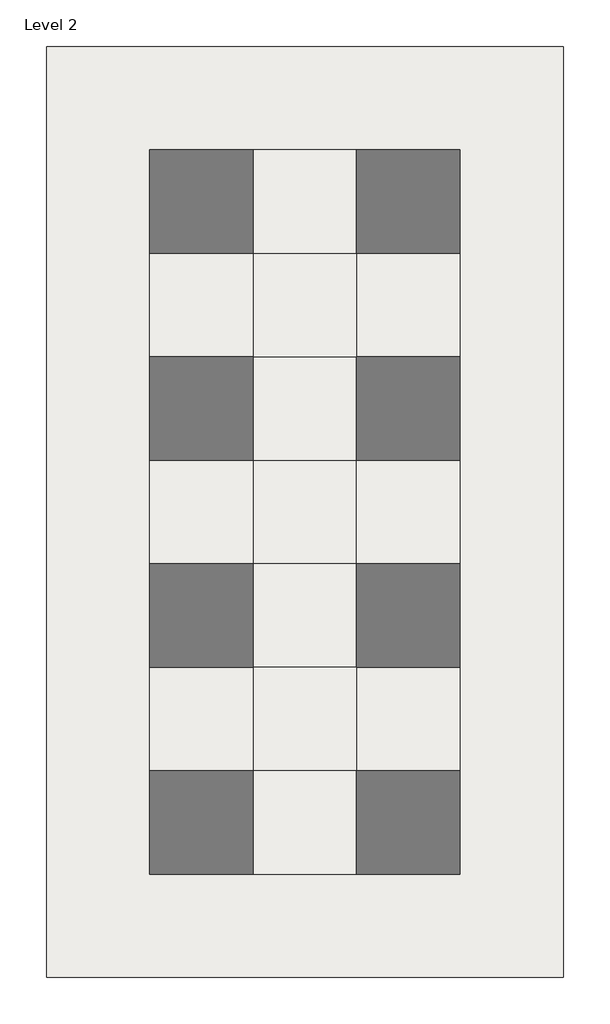
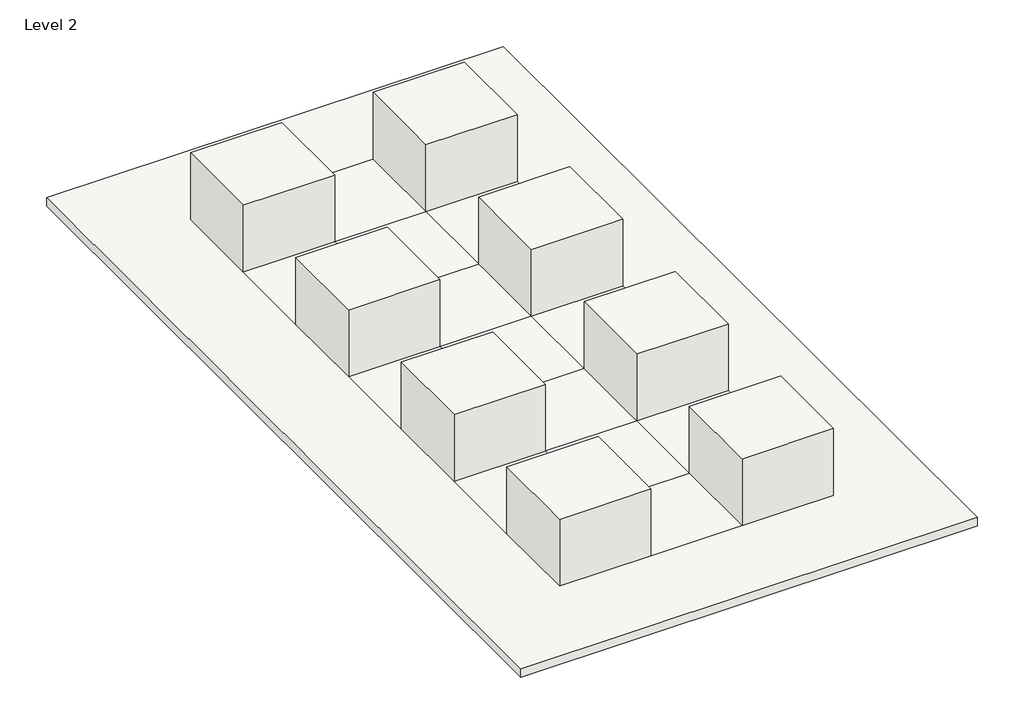
# One storey: 9 roofs.
# Revit data of these elements (continued)
# Materials (continued)
#   "Bauder_SeparationAndSlipLayer_BauderGREEN-PE-02": class "Unassigned", colour RGB 255 255 255, transparency 0, Mtrl_Author = "AM", Mtrl_AuthorizedBy = "bimstore", Mtrl_DistributedBy = "www.bimstore.co", Mtrl_AccessibilityPerformance = "n/a", Mtrl_AssetIdentifier = "Please record on commissioning", Mtrl_AssetType = "Fixed", Mtrl_BarCode = "Please record on commissioning", Mtrl_ClassificationName = "Uniclass2015", Mtrl_ClassificationValue = "n/a", Mtrl_CodePerformance = "n/a", Mtrl_Color = "n/a", Mtrl_Constituents = "n/a", Mtrl_CreatedBy = "technical@bauder.co.uk", Mtrl_CreatedOn = "2023-02-10 T00:00:00", Mtrl_DocumentationCertificates = "https://www.bimstore.co/products/intensive-green-roof-system/document/product-certificates", Mtrl_DocumentationInstallationGuide = "https://www.bimstore.co/products/intensive-green-roof-system/document/installation-guide", Mtrl_DocumentationLiterature = "https://www.bimstore.co/products/intensive-green-roof-system/document/product-literature", Mtrl_DocumentationMaintenance = "https://www.bimstore.co/products/intensive-green-roof-system/document/maintenance-information", Mtrl_DocumentationTechnical = "https://www.bimstore.co/products/intensive-green-roof-system/document/technical-data-sheet", Mtrl_DurationUnit = "Year", Mtrl_Features = "n/a", Mtrl_Finish = "n/a", Mtrl_Grade = "n/a", Mtrl_InstallationDate = "Please record on commissioning", Mtrl_ManufacturerName = "Bauder Ltd", Mtrl_Material = "n/a", Mtrl_ModelNumber = "BauderGREEN-PE-02", Mtrl_ModelReference = "Separation And Slip Layer", Mtrl_ProductionYear = "2023", Mtrl_ReferencedStandard = "n/a", Mtrl_Shape = "n/a", Mtrl_Size = "n/a", Mtrl_SpareParts = "n/a", Mtrl_TypeName = "BauderGREEN-PE-02", Mtrl_WarrantyDescription = "As part of Bauder system guarantee, per specification", Mtrl_WarrantyDurationUnit = "Year", Mtrl_WarrantyGuarantorLabor = "n/a", Mtrl_WarrantyGuarantorParts = "technical@bauder.co.uk", Mtrl_WarrantyStartDate = "Please record on commissioning", Mtrl_IfcExportAs = "IfcRoofType", Mtrl_IfcExportType = "FLAT_ROOF", Mtrl_BIMObjectName = "Bauder_SeparationAndSlipLayer_BauderGREEN-PE-02", Mtrl_NBSDescription = "n/a", Mtrl_NBSNote = "n/a", Mtrl_NBSObjectName = "n/a", Mtrl_NBSOfficeMasterTag = "n/a", Mtrl_NBSReference = "Q37", Mtrl_Ballast = "n/a", Mtrl_CarrierMembraneAttachment = "n/a", Mtrl_CarrierMembraneFixing = "n/a", Mtrl_CarrierMembraneType = "n/a", Mtrl_Certification = "Comply with GRO Green Roof Code of Practice and FLL Standards", Mtrl_DetailWorkAncillaryItems = "Detail as per project specific Bauder Specification", Mtrl_DetailWorkCoverStrips = "Detail as per project specific Bauder Specification", Mtrl_DetailWorkFlashings = "Detail as per project specific Bauder Specification", Mtrl_DetailWorkSkirtingsAndUpstands = "Detail as per project specific Bauder Specification", Mtrl_DetailWorkWeltedDrips = "Detail as per project specific Bauder Specification", Mtrl_EdgeRestraints = "Detail as per project specific Bauder Specification", Mtrl_FillToPerimeterUpstands = "n/a", Mtrl_FilterLayer = "n/a", Mtrl_InsulationAttachment = "As per project specific Bauder Specification", Mtrl_InsulationFixing = "As per project specific Bauder Specification", Mtrl_InsulationType = "As per project specific Bauder Specification", Mtrl_IsolatingLayer = "n/a", Mtrl_LiquidAppliedWaterproofCoatingReinforcement = "As per project specific Bauder Specification", Mtrl_LiquidAppliedWaterproofCoatingSurfaceTreatment = "As per project specific Bauder Specification", Mtrl_LiquidAppliedWaterproofCoatingType = "As per project specific Bauder Specification", Mtrl_LiquidAppliedWaterproofCoatingWearingCourse = "As per project specific Bauder Specification", Mtrl_LowerProtectionLayer = "n/a", Mtrl_MoistureControlDrainageAncillaries = "n/a", Mtrl_MoistureControlDrainageLayer = "n/a", Mtrl_MoistureControlFilterMembrane = "n/a", Mtrl_MoistureControlMoistureRetentionMat = "n/a", Mtrl_OverlayFixing = "n/a", Mtrl_OverlayType = "n/a", Mtrl_PlantingSystemsAntierosionMat = "n/a", Mtrl_PlantingSystemsPlantingMedium = "As per project specific Bauder Specification", Mtrl_PlantingSystemsVegetation = "As per project specific Bauder Specification", Mtrl_PlantingSystemsVegetationBarrier = "As per project specific Bauder Specification", Mtrl_PreparationExistingSubstrates = "n/a", Mtrl_PreparationHorizontalWork = "n/a", Mtrl_PreparationSkirtingsAndVerticalWork = "n/a", Mtrl_ProjectSpecificationAndDesign = "This BIM Object must be supported by a project specific specification from Bauder, incorporating system build-up, detail design and performance calculations if a full Bauder system warranty is required. Please contact your local Bauder Representative or technical@bauder.co.uk", Mtrl_ProtectionLayer = "n/a", Mtrl_ProtectionProtectionLayer = "n/a", Mtrl_ProtectionRootBarrier = "As per project specific Bauder Specification", Mtrl_ProtectionSeparationLayer = "n/a", Mtrl_SeparatingLayer = "n/a", Mtrl_SurfaceProtection = "n/a", Mtrl_SystemAccessories = "n/a", Mtrl_SystemManufacturer = "Bauder Ltd", Mtrl_Update = "1900-12-31 T23:59:59", Mtrl_UpperProtectionLayer = "n/a", Mtrl_VapourControlLayerAttachment = "As per project specific Bauder Specification", Mtrl_VapourControlLayerAttachment_Bauder = "As per project specific Bauder Specification", Mtrl_VapourControlLayerType = "As per project specific Bauder Specification", Mtrl_WarrantyConsiderations = "All guarantees available for this system are subject to the works being carried out in accordance with the Bauder specification and being installed by a Bauder Approved installer. For full details and further information regarding guarantees and alternative systems please contact your local Bauder Representative or technical@bauder.co.uk", Mtrl_WaterproofCoveringAccessories = "As per project specific Bauder Specification", Mtrl_WaterproofCoveringAttachment = "As per project specific Bauder Specification", Mtrl_WaterproofCoveringFirstLayerAttachment = "As per project specific Bauder Specification", Mtrl_WaterproofCoveringFirstLayerType = "As per project specific Bauder Specification", Mtrl_WaterproofCoveringIntermediateLayerAttachment = "As per project specific Bauder Specification", Mtrl_WaterproofCoveringIntermediateLayerType = "As per project specific Bauder Specification", Mtrl_WaterproofCoveringJoints = "As per project specific Bauder Specification", Mtrl_WaterproofCoveringTopLayerAttachment = "As per project specific Bauder Specification", Mtrl_WaterproofCoveringTopLayerType = "As per project specific Bauder Specification", Mtrl_WaterproofCoveringType = "As per project specific Bauder Specification", Cost = 0, Mtrl_ReplacementCost = 0, Mtrl_NominalDepth = 0.4 mm, Mtrl_NominalHeight = 0 mm, Mtrl_NominalLength = 0 mm, Mtrl_BimSpecGuid = 0, Mtrl_BSBibleVersion = 17, Mtrl_CurrentRevision = 2, Mtrl_ExpectedLife = 0, Mtrl_SerialNumber = 0, Mtrl_WarrantyDurationLabor = 0, Mtrl_WarrantyDurationParts = 0
